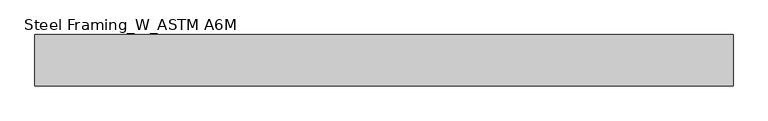
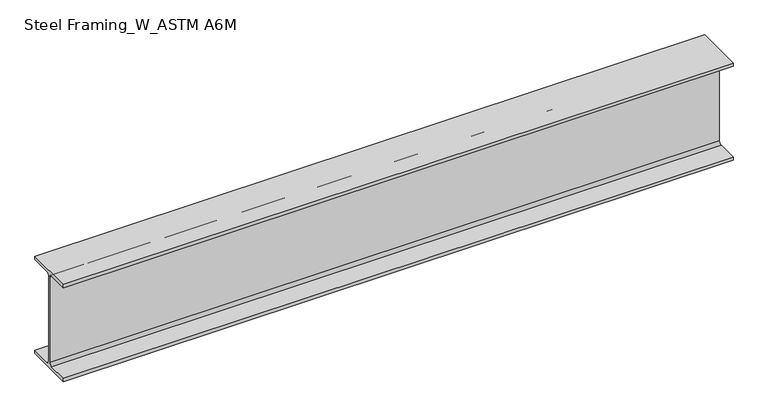
"""IFC4 building model written with IfcOpenShell, lengths in millimetres: beam geometry, Steel Framing_W_ASTM A6M : H_SB_AR_S02_W360x51_G3."""

from ifc_helpers import new_model, si_unit, point, frame, frame_2d, origin, place, context, project, spatial, polyline, circle_curve, trimmed, segment, composite_curve, outline, extrude, source, transform, mapped, element, save


def steel_framing_w_astm_a6m_44bd27a9(model_context):
    return source(origin(), model_context, "Body", "SweptSolid", [
        extrude(outline(composite_curve([segment(polyline([(85.5, -166.4), (85.5, -178.0), (-85.5, -178.0), (-85.5, -166.4), (-13.72, -166.4)]), True, "CONTINUOUS"), segment(trimmed(circle_curve(frame_2d((-13.72, -156.3)), 10.1), [point((-13.72, -166.4))], [point((-3.62, -156.3))], True, "CARTESIAN"), True, "CONTINUOUS"), segment(polyline([(-3.62, -156.3), (-3.62, 156.3)]), True, "CONTINUOUS"), segment(trimmed(circle_curve(frame_2d((-13.72, 156.3)), 10.1), [point((-3.62, 156.3))], [point((-13.72, 166.4))], True, "CARTESIAN"), True, "CONTINUOUS"), segment(polyline([(-13.72, 166.4), (-85.5, 166.4), (-85.5, 178.0), (85.5, 178.0), (85.5, 166.4), (13.72, 166.4)]), True, "CONTINUOUS"), segment(trimmed(circle_curve(frame_2d((13.72, 156.3)), 10.1), [point((13.72, 166.4))], [point((3.62, 156.3))], True, "CARTESIAN"), True, "CONTINUOUS"), segment(polyline([(3.62, 156.3), (3.62, -156.3)]), True, "CONTINUOUS"), segment(trimmed(circle_curve(frame_2d((13.72, -156.3)), 10.1), [point((3.62, -156.3))], [point((13.72, -166.4))], True, "CARTESIAN"), True, "CONTINUOUS"), segment(polyline([(13.72, -166.4), (85.5, -166.4)]), True, "CONTINUOUS")], self_intersect=False)), frame((-1003.8, 0.0, 0.0), z_axis=(1.0, 0.0, 0.0), x_axis=(0.0, 1.0, 0.0)), (0.0, 0.0, 1.0), 2320.8),
    ])


if __name__ == "__main__":
    model = new_model("IFC4")
    model_context = context("Model", 3, world=origin())
    ifc_project = project(units=[si_unit("LENGTHUNIT", "METRE", prefix="MILLI")], contexts=[model_context])
    site = spatial("IfcSite", under=ifc_project)
    building = spatial("IfcBuilding", under=site)
    placement = place(None, origin())
    steel_framing_w_astm_a6m_shape = steel_framing_w_astm_a6m_44bd27a9(model_context)
    element("IfcBeam", 1, ObjectType="Steel Framing_W_ASTM A6M : H_SB_AR_S02_W360x51_G3", at=placement, inside=building, context=model_context, shape_type="MappedRepresentation", body=[
        mapped(steel_framing_w_astm_a6m_shape, transform((0.0, 0.0, 0.0), x_axis=(1.0, 0.0, 0.0), y_axis=(0.0, 1.0, 0.0), z_axis=(0.0, 0.0, 1.0))),
    ])
    save(model, "model.ifc")

# Revit data of these elements
# Type "Steel Framing_W_ASTM A6M : H_SB_AR_S02_W360x51_G3"
#   Type Mark = "G3"
#   Section Name Key = "W14x34"
#   Width = 17.1 cm
#   Web Thickness = 0.724 cm
#   Web Fillet = 1.01 cm
#   Warping Constant = 287000.0 cm⁶
#   Torsional Moment of Inertia = 23.70 cm⁴
#   Section Area = 64.5 cm²
#   Plastic Modulus weak axis = 174.0 cm³
#   Plastic Modulus strong axis = 895.0 cm³
#   Perimeter = 1.36 m²/m
#   Nominal Weight = 51.00 kgf/m
#   Moment of Inertia weak axis = 970.00 cm⁴
#   Moment of Inertia strong axis = 14200.00 cm⁴
#   Height = 35.6 cm
#   Flange Thickness = 1.16 cm
#   Elastic Modulus weak axis = 113.0 cm³
#   Elastic Modulus strong axis = 796.0 cm³
#   Centroid Vertical = 17.8 cm
#   Centroid Horizontal = 8.55 cm
#   Length [instance default] = 1500 mm
#   Structural Material [instance default] = Steel, 45-345
#   Bolt Spacing = 0
#   Assembly Code = ""
# Element 1 (IfcBeam, "Steel Framing_W_ASTM A6M : H_SB_AR_S02_W360x51_G3")
#   Materials on its faces: "Steel, 45-345"
# Materials
#   "Steel, 45-345": class "Metal", colour RGB 189 187 185, transparency 0, Description = "Steel 345 MPa", Cost = 0
